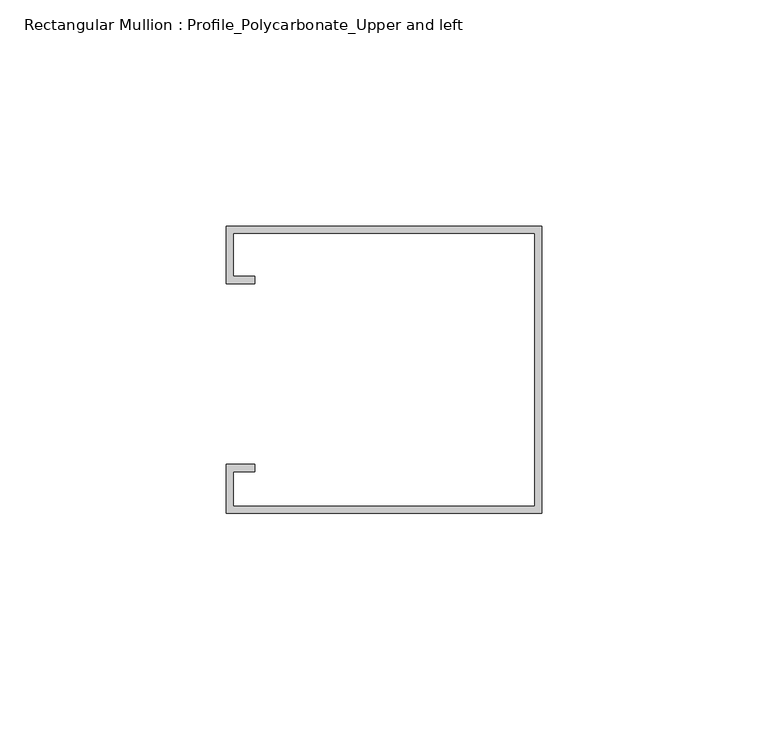
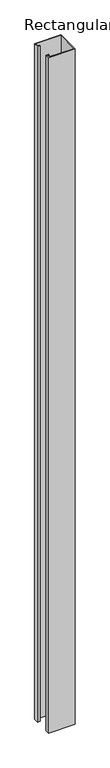
"""IFC4 building model written with IfcOpenShell, lengths in millimetres: member geometry, Rectangular Mullion : Profile_Polycarbonate_Upper and left."""

from ifc_helpers import new_model, si_unit, frame, origin, place, context, project, spatial, polyline, outline, extrude, source, transform, mapped, element, save


def rectangular_mullion_profile_polycarbonate_upper_and_left_d75ed421(model_context):
    return source(origin(), model_context, "Body", "SweptSolid", [
        extrude(outline(polyline([(0.0, 32.7), (0.0, -30.8), (-69.85, -30.8), (-69.85, -20.0), (-63.5, -20.0), (-63.5, -21.5875), (-68.2625, -21.5875), (-68.2625, -29.2125), (-1.5875, -29.2125), (-1.5875, 31.1125), (-68.2625, 31.1125), (-68.2625, 21.5875), (-63.5, 21.5875), (-63.5, 20.0), (-69.85, 20.0), (-69.85, 32.7), (0.0, 32.7)])), frame((0.0, 0.0, -1879.6), z_axis=(0.0, 0.0, 1.0), x_axis=(1.0, 0.0, 0.0)), (0.0, 0.0, 1.0), 1879.6),
    ])


if __name__ == "__main__":
    model = new_model("IFC4")
    model_context = context("Model", 3, world=origin())
    ifc_project = project(units=[si_unit("LENGTHUNIT", "METRE", prefix="MILLI")], contexts=[model_context])
    site = spatial("IfcSite", under=ifc_project)
    building = spatial("IfcBuilding", under=site)
    placement = place(None, origin())
    rectangular_mullion_profile_polycarbonate_upper_and_left_shape = rectangular_mullion_profile_polycarbonate_upper_and_left_d75ed421(model_context)
    element("IfcMember", 1, ObjectType="Rectangular Mullion : Profile_Polycarbonate_Upper and left", at=placement, inside=building, context=model_context, shape_type="MappedRepresentation", body=[
        mapped(rectangular_mullion_profile_polycarbonate_upper_and_left_shape, transform((0.0, 0.0, 0.0), x_axis=(1.0, 0.0, 0.0), y_axis=(0.0, 1.0, 0.0), z_axis=(0.0, 0.0, 1.0))),
    ])
    save(model, "model.ifc")

# Revit data of these elements
# Type "Rectangular Mullion : Profile_Polycarbonate_Upper and left"
#   built-in parameter 1007322 = 0.208333 (stored number, unit not read)
#   built-in parameter 1007321 = 0.00520833 (stored number, unit not read)
#   built-in parameter 1007320 = 0 (stored number, unit not read)
# Element 1 (IfcMember, "Rectangular Mullion : Profile_Polycarbonate_Upper and left")
#   Materials on its faces: "ALUMINUM PROFILE AT POLYCARBONATE PANEL"
# Materials
#   "ALUMINUM PROFILE AT POLYCARBONATE PANEL": class "Metal", colour RGB 244 244 244, transparency 0, Description = "Aluminum 6061", Cost = 0
